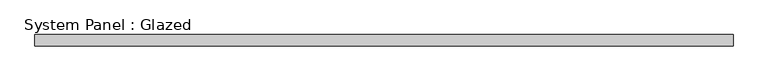
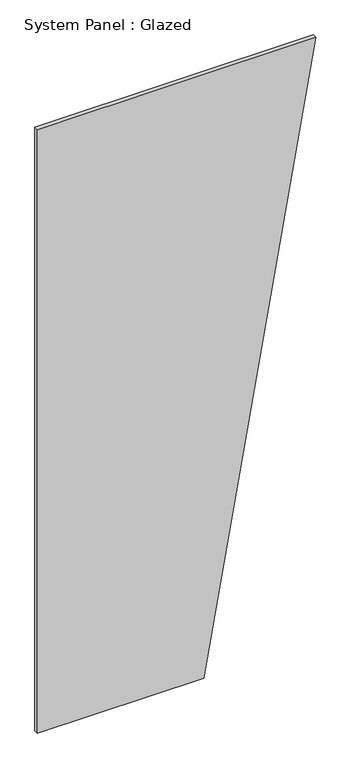
"""IFC4 building model written with IfcOpenShell, lengths in millimetres: plate geometry, System Panel : Glazed."""

import ifcopenshell
import ifcopenshell.guid

model = None  # the IFC model being written
_history = None  # IfcOwnerHistory: only IFC2X3 demands one
_inside = {}  # id of a spatial element -> (the spatial element, [elements in it])
_under = {}  # id of a project, library or spatial element -> (it, [spatial elements below it])
_declared = {}  # id of a project -> (the project, [libraries it declares])
_typed = {}  # id of a type object -> (the type object, [elements of that type])
_made_of = {}  # id of a material, layer set ... -> (it, [elements and type objects made of it])


def new_model(schema):
    """Start an empty IFC model of exactly this schema.

    Asked for "IFC4X3", IfcOpenShell would pick the latest addendum, in which some entities
    have other attributes; the version numbers below select the first issue.
    IFC2X3 requires an IfcOwnerHistory on every rooted entity: one is made here for all.
    """
    global model, _history
    if schema == "IFC4X3":
        model = ifcopenshell.file(schema_version=(4, 3, 0, 0))
    else:
        model = ifcopenshell.file(schema=schema)
    _inside.clear()
    _under.clear()
    _declared.clear()
    _typed.clear()
    _made_of.clear()
    _history = None
    if model.schema == "IFC2X3":
        org = make("IfcOrganization", Name="unknown")
        user = make(
            "IfcPersonAndOrganization",
            ThePerson=make("IfcPerson", FamilyName="unknown"),
            TheOrganization=org,
        )
        app = make(
            "IfcApplication",
            ApplicationDeveloper=org,
            Version="unknown",
            ApplicationFullName="unknown",
            ApplicationIdentifier="unknown",
        )
        _history = make(
            "IfcOwnerHistory",
            OwningUser=user,
            OwningApplication=app,
            ChangeAction="ADDED",
            CreationDate=0,
        )
    return model


def make(cls, **values):
    """One entity of the class cls with the attributes given. An attribute that is None is left unset."""
    return model.create_entity(
        cls, **{name: value for name, value in values.items() if value is not None}
    )


def rooted(cls, **values):
    """An entity with a GlobalId (a new one), such as an element, a storey or a relation."""
    return make(cls, GlobalId=ifcopenshell.guid.new(), OwnerHistory=_history, **values)


def si_unit(unit_type, name, prefix=None):
    """IfcSIUnit, for example si_unit("LENGTHUNIT", "METRE", prefix="MILLI")."""
    return make("IfcSIUnit", UnitType=unit_type, Prefix=prefix, Name=name)


def assignment(units):
    """IfcUnitAssignment: the units of a project."""
    return None if units is None else make("IfcUnitAssignment", Units=units)


def point(xyz):
    """IfcCartesianPoint."""
    return None if xyz is None else make("IfcCartesianPoint", Coordinates=xyz)


def direction(xyz):
    """IfcDirection."""
    return None if xyz is None else make("IfcDirection", DirectionRatios=xyz)


def frame(location, z_axis=None, x_axis=None):
    """IfcAxis2Placement3D, a coordinate frame: its origin and axes. An axis left out is left unset."""
    return make(
        "IfcAxis2Placement3D",
        Location=point(location),
        Axis=direction(z_axis),
        RefDirection=direction(x_axis),
    )


def origin():
    """The frame at (0, 0, 0) with its axes left unset."""
    return frame((0.0, 0.0, 0.0))


def place(relative_to, where):
    """IfcLocalPlacement: puts the frame where relative to a parent placement (None: the world)."""
    return make(
        "IfcLocalPlacement", PlacementRelTo=relative_to, RelativePlacement=where
    )


def context(
    kind, dimensions, precision=None, world=None, true_north=None, identifier=None
):
    """IfcGeometricRepresentationContext, for example the 3D "Model" context."""
    return make(
        "IfcGeometricRepresentationContext",
        ContextIdentifier=identifier,
        ContextType=kind,
        CoordinateSpaceDimension=dimensions,
        Precision=precision,
        WorldCoordinateSystem=world,
        TrueNorth=true_north,
    )


def project(units=None, contexts=None):
    """IfcProject with its units and contexts."""
    return rooted(
        "IfcProject",
        Name="project",
        RepresentationContexts=contexts,
        UnitsInContext=assignment(units),
    )


def spatial(cls, under=None, at=None, **own):
    """A site, building, storey or space (cls), placed at a placement, below another one or the project."""
    s = rooted(cls, ObjectPlacement=at, **own)
    if under is not None:
        _under.setdefault(under.id(), (under, []))[1].append(s)
    return s


def polyline(points):
    """IfcPolyline through the points."""
    return make("IfcPolyline", Points=[point(p) for p in points])


def outline(outer, holes=None, kind="AREA"):
    """IfcArbitraryClosedProfileDef: a profile drawn as a closed curve; with holes, ...WithVoids."""
    if holes is None:
        return make("IfcArbitraryClosedProfileDef", ProfileType=kind, OuterCurve=outer)
    return make(
        "IfcArbitraryProfileDefWithVoids",
        ProfileType=kind,
        OuterCurve=outer,
        InnerCurves=holes,
    )


def extrude(swept, where, along, depth):
    """IfcExtrudedAreaSolid: the profile swept, set in the frame where, extruded along a direction by depth."""
    return make(
        "IfcExtrudedAreaSolid",
        SweptArea=swept,
        Position=where,
        ExtrudedDirection=direction(along),
        Depth=depth,
    )


def shape(context_of_items, identifier, shape_type, items):
    """IfcShapeRepresentation: the items that make up one representation, for example the "Body"."""
    return make(
        "IfcShapeRepresentation",
        ContextOfItems=context_of_items,
        RepresentationIdentifier=identifier,
        RepresentationType=shape_type,
        Items=items,
    )


def source(mapping_origin, context_of_items, identifier, shape_type, items):
    """IfcRepresentationMap: a shape defined once, which mapped items show again and again."""
    return make(
        "IfcRepresentationMap",
        MappingOrigin=mapping_origin,
        MappedRepresentation=shape(context_of_items, identifier, shape_type, items),
    )


def transform(
    local_origin,
    x_axis=None,
    y_axis=None,
    z_axis=None,
    scale=None,
    scale2=None,
    scale3=None,
    uniform=True,
):
    """IfcCartesianTransformationOperator3D, or its non-uniform kind. x_axis, y_axis, z_axis: its Axis1, 2, 3."""
    if uniform:
        return make(
            "IfcCartesianTransformationOperator3D",
            Axis1=direction(x_axis),
            Axis2=direction(y_axis),
            LocalOrigin=point(local_origin),
            Scale=scale,
            Axis3=direction(z_axis),
        )
    return make(
        "IfcCartesianTransformationOperator3DnonUniform",
        Axis1=direction(x_axis),
        Axis2=direction(y_axis),
        LocalOrigin=point(local_origin),
        Scale=scale,
        Axis3=direction(z_axis),
        Scale2=scale2,
        Scale3=scale3,
    )


def mapped(mapping_source, mapping_target):
    """IfcMappedItem: shows the shape of a source again, moved by a transform."""
    return make(
        "IfcMappedItem", MappingSource=mapping_source, MappingTarget=mapping_target
    )


def made_of(thing, what):
    """Note that an element or type object is made of a material, layer set ...; save() writes the relation."""
    if what is not None:
        _made_of.setdefault(what.id(), (what, []))[1].append(thing)
    return thing


def element(
    cls,
    number,
    at=None,
    inside=None,
    cuts=None,
    type_object=None,
    material=None,
    context=None,
    identifier="Body",
    shape_type=None,
    held_by="IfcProductDefinitionShape",
    body=None,
    shapes=None,
    **own,
):
    """One element of the class cls, such as IfcWall. Its Tag is "e" and its number.

    at: its placement. inside: the storey or other place that contains it. cuts: it is an
    opening in that element (IfcRelVoidsElement). A single representation is given by context,
    identifier, shape_type and body (its items); several are given by shapes. held_by: the class
    of the entity that holds the representations. save() writes the other relations.
    """
    e = rooted(cls, Tag="e%d" % number, ObjectPlacement=at, **own)
    if body is not None:
        shapes = [shape(context, identifier, shape_type, body)]
    if shapes is not None:
        e.Representation = make(held_by, Representations=shapes)
    if inside is not None:
        _inside.setdefault(inside.id(), (inside, []))[1].append(e)
    if cuts is not None:
        rooted(
            "IfcRelVoidsElement", RelatingBuildingElement=cuts, RelatedOpeningElement=e
        )
    if type_object is not None:
        _typed.setdefault(type_object.id(), (type_object, []))[1].append(e)
    return made_of(e, material)


def aggregate(whole, parts):
    """IfcRelAggregates: a whole, such as a stair, and the parts it consists of."""
    return rooted("IfcRelAggregates", RelatingObject=whole, RelatedObjects=parts)


def save(model, path):
    """Write the relations noted so far, then the file.

    IfcRelAggregates (storeys below a building ...), IfcRelContainedInSpatialStructure (elements
    in a storey), IfcRelDefinesByType, IfcRelAssociatesMaterial and IfcRelDeclares: one each for
    every whole, place, type object, material and project.
    """
    for whole, parts in _under.values():
        aggregate(whole, parts)
    for where, things in _inside.values():
        rooted(
            "IfcRelContainedInSpatialStructure",
            RelatedElements=things,
            RelatingStructure=where,
        )
    for kind, things in _typed.values():
        rooted("IfcRelDefinesByType", RelatedObjects=things, RelatingType=kind)
    for what, things in _made_of.values():
        rooted("IfcRelAssociatesMaterial", RelatedObjects=things, RelatingMaterial=what)
    for by, libraries in _declared.values():
        rooted("IfcRelDeclares", RelatingContext=by, RelatedDefinitions=libraries)
    model.write(path)


def system_panel_glazed_2bad594a(model_context):
    return source(origin(), model_context, "Body", "SweptSolid", [
        extrude(outline(polyline([(0.0, -797.3917397), (0.0, 154.912342), (3657.6, 797.3917397), (3657.6, -797.3917397), (0.0, -797.3917397)])), frame((0.0, -44.45, 0.0), z_axis=(0.0, 1.0, 0.0), x_axis=(0.0, 0.0, 1.0)), (0.0, 0.0, 1.0), 25.4),
    ])


if __name__ == "__main__":
    model = new_model("IFC4")
    model_context = context("Model", 3, world=origin())
    ifc_project = project(units=[si_unit("LENGTHUNIT", "METRE", prefix="MILLI")], contexts=[model_context])
    site = spatial("IfcSite", under=ifc_project)
    building = spatial("IfcBuilding", under=site)
    placement = place(None, origin())
    system_panel_glazed_shape = system_panel_glazed_2bad594a(model_context)
    element("IfcPlate", 1, ObjectType="System Panel : Glazed", at=placement, inside=building, context=model_context, shape_type="MappedRepresentation", body=[
        mapped(system_panel_glazed_shape, transform((0.0, 0.0, 0.0), x_axis=(1.0, 0.0, 0.0), y_axis=(0.0, 1.0, 0.0), z_axis=(0.0, 0.0, 1.0))),
    ])
    save(model, "model.ifc")

# Revit data of these elements
# Type "System Panel : Glazed"
#   Construction Type Id = "GSP4R"
#   Analytic Construction = "1/8 in Pilkington single glazing"
#   Visual Light Transmittance = 0.9
#   Solar Heat Gain Coefficient = 0.86
#   Heat Transfer Coefficient (U) = 1.18115 BTU/(h·ft²·°F)
#   Define Thermal Properties by = 1
# Element 1 (IfcPlate, "System Panel : Glazed")
#   Materials on its faces: "Glass"
# Materials
#   "Glass": class "Glass", colour RGB 0 128 192, transparency 0.75, Description = "Soda Lime Glass", Cost = 0
